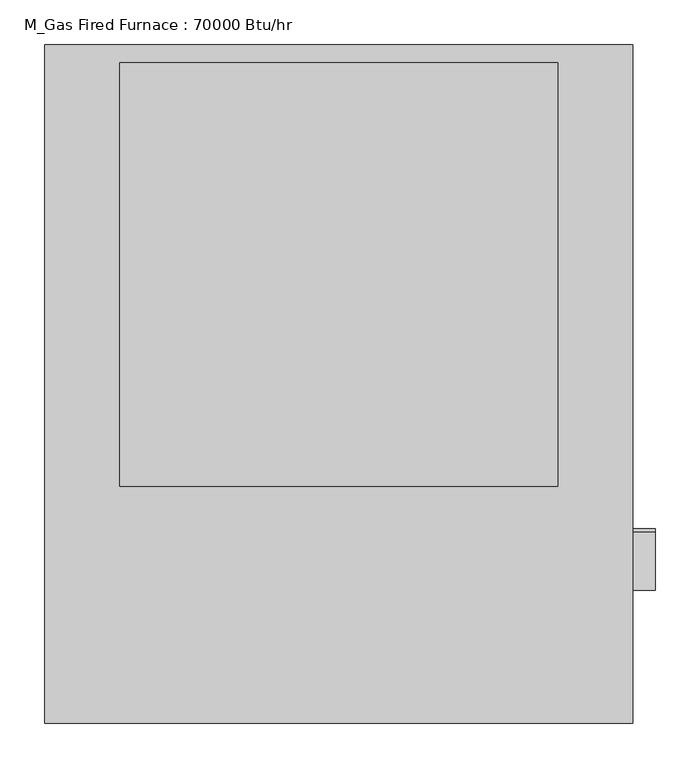
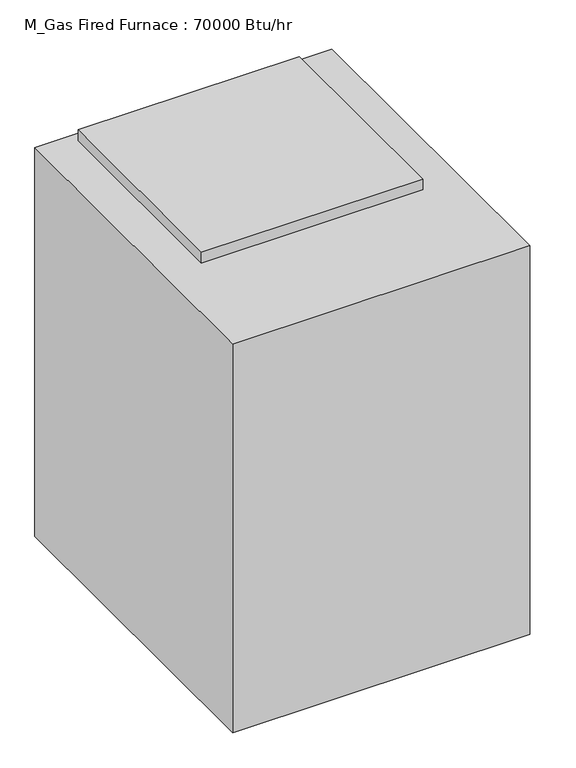
"""IFC4 building model written with IfcOpenShell, lengths in millimetres: proxy geometry, M_Gas Fired Furnace : 70000 Btu/hr."""

from ifc_helpers import new_model, si_unit, frame, origin, place, context, project, spatial, circle_curve, source, transform, mapped, element, save
from ifc_brep_helpers import plane_surface, cylinder_surface, advanced_brep


def m_gas_fired_furnace_70000_btu_hr_1f9757d0(model_context):
    return source(origin(), model_context, "Body", "AdvancedBrep", [
        advanced_brep(
        [(0.0, 0.0, 914.4), (-660.4, 0.0, 914.4), (-660.4, -762.0, 914.4), (0.0, -762.0, 914.4), (-576.2, -20.6375, 914.4), (-84.2, -20.6375, 914.4), (-84.2, -495.6375, 914.4), (-576.2, -495.6375, 914.4), (0.0, 0.0, 0.0), (0.0, -762.0, 0.0), (-660.4, -762.0, 0.0), (-660.4, 0.0, 0.0), (0.0, -547.4666667, 844.55), (0.0, -612.4666667, 844.55), (0.0, -572.4666667, 774.7), (0.0, -587.4666667, 774.7), (0.0, -543.7625, 463.55), (0.0, -608.7625, 463.55), (25.4, -612.4666667, 844.55), (25.4, -547.4666667, 844.55), (25.4, -587.4666667, 774.7), (25.4, -572.4666667, 774.7), (25.4, -608.7625, 463.55), (25.4, -543.7625, 463.55), (-84.2, -20.6375, 939.8), (-576.2, -20.6375, 939.8), (-576.2, -495.6375, 939.8), (-84.2, -495.6375, 939.8)],
        [
            (0, 1),
            (1, 2),
            (2, 3),
            (3, 0),
            (4, 5),
            (5, 6),
            (6, 7),
            (7, 4),
            (8, 9),
            (9, 10),
            (10, 11),
            (11, 8),
            (0, 8),
            (11, 1),
            (10, 2),
            (9, 3),
            (12, 13, circle_curve(frame((0.0, -579.9666667, 844.55), z_axis=(-1.0, 0.0, 0.0), x_axis=(0.0, 1.0, 0.0)), 32.5)),
            (13, 12, circle_curve(frame((0.0, -579.9666667, 844.55), z_axis=(-1.0, 0.0, 0.0), x_axis=(0.0, 1.0, 0.0)), 32.5)),
            (14, 15, circle_curve(frame((0.0, -579.9666667, 774.7), z_axis=(-1.0, 0.0, 0.0), x_axis=(0.0, 1.0, 0.0)), 7.5)),
            (15, 14, circle_curve(frame((0.0, -579.9666667, 774.7), z_axis=(-1.0, 0.0, 0.0), x_axis=(0.0, 1.0, 0.0)), 7.5)),
            (16, 17, circle_curve(frame((0.0, -576.2625, 463.55), z_axis=(-1.0, 0.0, 0.0), x_axis=(0.0, 1.0, 0.0)), 32.5)),
            (17, 16, circle_curve(frame((0.0, -576.2625, 463.55), z_axis=(-1.0, 0.0, 0.0), x_axis=(0.0, 1.0, 0.0)), 32.5)),
            (18, 19, circle_curve(frame((25.4, -579.9666667, 844.55), z_axis=(1.0, 0.0, 0.0), x_axis=(0.0, 1.0, 0.0)), 32.5)),
            (19, 18, circle_curve(frame((25.4, -579.9666667, 844.55), z_axis=(1.0, 0.0, 0.0), x_axis=(0.0, 1.0, 0.0)), 32.5)),
            (20, 21, circle_curve(frame((25.4, -579.9666667, 774.7), z_axis=(1.0, 0.0, 0.0), x_axis=(0.0, 1.0, 0.0)), 7.5)),
            (21, 20, circle_curve(frame((25.4, -579.9666667, 774.7), z_axis=(1.0, 0.0, 0.0), x_axis=(0.0, 1.0, 0.0)), 7.5)),
            (22, 23, circle_curve(frame((25.4, -576.2625, 463.55), z_axis=(1.0, 0.0, 0.0), x_axis=(0.0, 1.0, 0.0)), 32.5)),
            (23, 22, circle_curve(frame((25.4, -576.2625, 463.55), z_axis=(1.0, 0.0, 0.0), x_axis=(0.0, 1.0, 0.0)), 32.5)),
            (18, 13),
            (12, 19),
            (20, 15),
            (14, 21),
            (22, 17),
            (16, 23),
            (24, 25),
            (25, 26),
            (26, 27),
            (27, 24),
            (24, 5),
            (4, 25),
            (7, 26),
            (6, 27),
        ],
        [
            plane_surface(frame((-660.4, 0.0, 914.4), z_axis=(0.0, 0.0, 1.0), x_axis=(-1.0, 0.0, 0.0))),
            plane_surface(frame((-660.4, 0.0, 0.0), z_axis=(0.0, 0.0, -1.0), x_axis=(1.0, 0.0, 0.0))),
            plane_surface(frame((0.0, 0.0, 914.4), z_axis=(0.0, 1.0, 0.0), x_axis=(0.0, 0.0, -1.0))),
            plane_surface(frame((-660.4, 0.0, 914.4), z_axis=(-1.0, 0.0, 0.0), x_axis=(0.0, 0.0, -1.0))),
            plane_surface(frame((-660.4, -762.0, 914.4), z_axis=(0.0, -1.0, 0.0), x_axis=(0.0, 0.0, -1.0))),
            plane_surface(frame((0.0, -762.0, 914.4), z_axis=(1.0, 0.0, 0.0), x_axis=(0.0, 0.0, -1.0))),
            plane_surface(frame((25.4, -547.4666667, 844.55), z_axis=(1.0, 0.0, 0.0), x_axis=(0.0, 0.0, 1.0))),
            cylinder_surface(frame((0.0, -579.9666667, 844.55), z_axis=(1.0, 0.0, 0.0), x_axis=(0.0, 1.0, 0.0)), 32.5),
            cylinder_surface(frame((0.0, -579.9666667, 774.7), z_axis=(1.0, 0.0, 0.0), x_axis=(0.0, 1.0, 0.0)), 7.5),
            cylinder_surface(frame((0.0, -576.2625, 463.55), z_axis=(1.0, 0.0, 0.0), x_axis=(0.0, 1.0, 0.0)), 32.5),
            plane_surface(frame((-576.2, -20.6375, 939.8), z_axis=(0.0, 0.0, 1.0), x_axis=(-1.0, 0.0, 0.0))),
            plane_surface(frame((-84.2, -20.6375, 939.8), z_axis=(0.0, 1.0, 0.0), x_axis=(0.0, 0.0, -1.0))),
            plane_surface(frame((-576.2, -20.6375, 939.8), z_axis=(-1.0, 0.0, 0.0), x_axis=(0.0, 0.0, -1.0))),
            plane_surface(frame((-576.2, -495.6375, 939.8), z_axis=(0.0, -1.0, 0.0), x_axis=(0.0, 0.0, -1.0))),
            plane_surface(frame((-84.2, -495.6375, 939.8), z_axis=(1.0, 0.0, 0.0), x_axis=(0.0, 0.0, -1.0))),
        ],
        [
            (0, [[1, 2, 3, 4], [5, 6, 7, 8]]),
            (1, [[9, 10, 11, 12]]),
            (2, [[-1, 13, -12, 14]]),
            (3, [[-2, -14, -11, 15]]),
            (4, [[-3, -15, -10, 16]]),
            (5, [[-4, -16, -9, -13], [17, 18], [19, 20], [21, 22]]),
            (6, [[23, 24]]),
            (6, [[25, 26]]),
            (6, [[27, 28]]),
            (7, [[-23, 29, -17, 30]]),
            (7, [[-24, -30, -18, -29]]),
            (8, [[-25, 31, -19, 32]]),
            (8, [[-26, -32, -20, -31]]),
            (9, [[-27, 33, -21, 34]]),
            (9, [[-28, -34, -22, -33]]),
            (10, [[35, 36, 37, 38]]),
            (11, [[-35, 39, -5, 40]]),
            (12, [[-36, -40, -8, 41]]),
            (13, [[-37, -41, -7, 42]]),
            (14, [[-38, -42, -6, -39]]),
        ],
    ),
    ])


if __name__ == "__main__":
    model = new_model("IFC4")
    model_context = context("Model", 3, world=origin())
    ifc_project = project(units=[si_unit("LENGTHUNIT", "METRE", prefix="MILLI")], contexts=[model_context])
    site = spatial("IfcSite", under=ifc_project)
    building = spatial("IfcBuilding", under=site)
    placement = place(None, origin())
    m_gas_fired_furnace_70000_btu_hr_shape = m_gas_fired_furnace_70000_btu_hr_1f9757d0(model_context)
    element("IfcBuildingElementProxy", 1, Name="M_Gas Fired Furnace : 70000 Btu/hr", ObjectType="M_Gas Fired Furnace : 70000 Btu/hr", at=placement, inside=building, context=model_context, shape_type="MappedRepresentation", body=[
        mapped(m_gas_fired_furnace_70000_btu_hr_shape, transform((0.0, 0.0, 0.0), x_axis=(1.0, 0.0, 0.0), y_axis=(0.0, 1.0, 0.0), z_axis=(0.0, 0.0, 1.0))),
    ])
    save(model, "model.ifc")

# Revit data of these elements
# Project information
#   Project Issue Date = "Issue Date"
#   Project Status = "Project Status"
#   Client Name = "Owner"
#   Project Address = "Enter address here"
#   Project Name = "Lake Geneva"
#   Project Number = "Project Number"
# Type "M_Gas Fired Furnace : 70000 Btu/hr"
#   Type Mark = "GF-01"
#   Static Pressure = 2.000 in-wg
#   dd = 0' - 3.62598"
#   Vent Radius = 1.27953"
#   Vent Diameter = 2.55906"
#   Supply Air Width = 19.37008"
#   Supply Air Height = 18.70079"
#   Return Air Width = 19 1/2"
#   Return Air Height = 24.18898"
#   Output Capacity [instance default] = 93833.9 Btu/h
#   Gas Radius = 0.29528"
#   Gas Pressure Drop [instance default] = 0.00 psi
#   Gas Flow [instance default] = 0 GPM
#   Gas Diameter = 0.59055"
#   Furnace Width = 2' - 6"
#   Furnace Length = 2' - 2"
#   Furnace Height = 3' - 0"
#   Exhaust Air Pressure Drop [instance default] = 0.000 in-wg
#   Exhaust Air Flow [instance default] = 0 CFM
#   Combustion Air Radius = 1.27953"
#   Combustion Air Pressure Drop [instance default] = 0.00 psi
#   Combustion Air Flow [instance default] = 0 GPM
#   Combustion Air Diameter = 2.55906"
#   Air Pressure Drop [instance default] = 0.000 in-wg
#   Air Flow [instance default] = 2000.22 CFM
#   Material = none
# Element 1 (IfcBuildingElementProxy, "M_Gas Fired Furnace : 70000 Btu/hr")
#   Output Capacity = 70000 Btu/h
#   Air Flow = 2400 CFM
